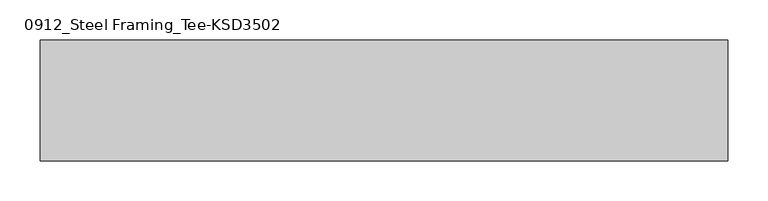
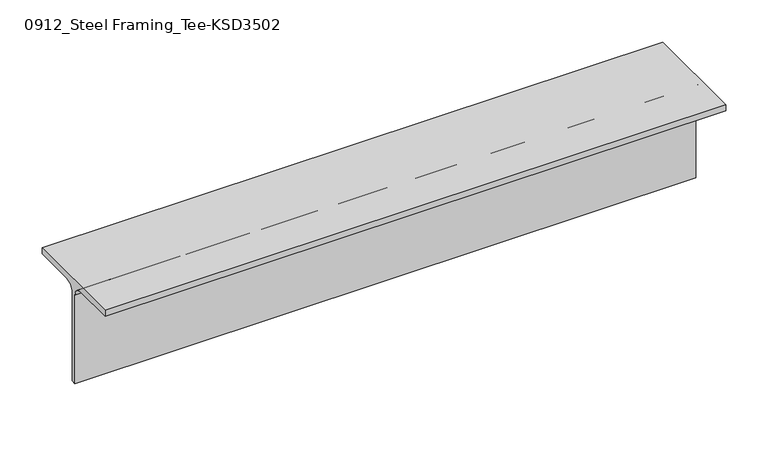
"""IFC4 building model written with IfcOpenShell, lengths in millimetres: member geometry, 0912_Steel Framing_Tee-KSD3502 : H_SB_ASB_CT-150x150x6.5x9."""

from ifc_helpers import new_model, si_unit, point, frame, frame_2d, origin, place, context, project, spatial, polyline, circle_curve, trimmed, segment, composite_curve, outline, extrude, source, transform, mapped, element, save


def member_0912_steel_framing_tee_ksd3502_a741d792(model_context):
    return source(origin(), model_context, "Body", "SweptSolid", [
        extrude(outline(composite_curve([segment(polyline([(75.0, 75.0), (75.0, 66.0), (16.25, 66.0)]), True, "CONTINUOUS"), segment(trimmed(circle_curve(frame_2d((16.25, 53.0)), 13.0), [point((16.25, 66.0))], [point((3.25, 53.0))], True, "CARTESIAN"), True, "CONTINUOUS"), segment(polyline([(3.25, 53.0), (3.25, -75.0), (-3.25, -75.0), (-3.25, 53.0)]), True, "CONTINUOUS"), segment(trimmed(circle_curve(frame_2d((-16.25, 53.0)), 13.0), [point((-3.25, 53.0))], [point((-16.25, 66.0))], True, "CARTESIAN"), True, "CONTINUOUS"), segment(polyline([(-16.25, 66.0), (-75.0, 66.0), (-75.0, 75.0), (75.0, 75.0)]), True, "CONTINUOUS")], self_intersect=False)), frame((-500.0, 0.0, 0.0), z_axis=(1.0, 0.0, 0.0), x_axis=(0.0, 1.0, 0.0)), (0.0, 0.0, 1.0), 853.0),
    ])


if __name__ == "__main__":
    model = new_model("IFC4")
    model_context = context("Model", 3, world=origin())
    ifc_project = project(units=[si_unit("LENGTHUNIT", "METRE", prefix="MILLI")], contexts=[model_context])
    site = spatial("IfcSite", under=ifc_project)
    building = spatial("IfcBuilding", under=site)
    placement = place(None, origin())
    member_0912_steel_framing_tee_ksd3502_shape = member_0912_steel_framing_tee_ksd3502_a741d792(model_context)
    element("IfcMember", 1, ObjectType="0912_Steel Framing_Tee-KSD3502 : H_SB_ASB_CT-150x150x6.5x9", at=placement, inside=building, context=model_context, shape_type="MappedRepresentation", body=[
        mapped(member_0912_steel_framing_tee_ksd3502_shape, transform((0.0, 0.0, 0.0), x_axis=(1.0, 0.0, 0.0), y_axis=(0.0, 1.0, 0.0), z_axis=(0.0, 0.0, 1.0))),
    ])
    save(model, "model.ifc")

# Revit data of these elements
# Type "0912_Steel Framing_Tee-KSD3502 : H_SB_ASB_CT-150x150x6.5x9"
#   H_WM Code_1 = "S01AA003-00001 | Main Steel Structure Fabrication Work | Shelter/Building | Light Steel - Standard (30KG/M>Weight) | Material: (   )"
#   H_WM Code_2 = "S03AA029-00001 | Main Steel Structure Erection Work | Shelter/Building | Light Steel (30KG/M>Weight) | Material: (   )"
#   H_WM Code_3 = "S01AA010-00001 | Main Steel Structure Fabrication Work | Shelter/Building | Steel Painting/Coating | for Non-Fireproofed Steel Surface, Surface Preparation, Primer, Second & Final Coat | Material: (   )"
#   H_Q'ty Cal Type Tag = "SB-Q2"
#   Width = 15.0 cm
#   Web Thickness = 0.65 cm
#   Web Fillet = 1.3 cm
#   Section Area = 23.39 cm²
#   Perimeter = 0.60 m²/m
#   Nominal Weight = 18.40 kgf/m
#   Height = 15.0 cm
#   Flange Thickness = 0.9 cm
#   Centroid Vertical = 7.5 cm
#   Centroid Horizontal = 7.5 cm
#   Length [instance default] = 1.5000 m
#   Structural Material [instance default] = Steel, 45-345
#   Warping Constant = (empty or 0)
#   Torsional Moment of Inertia = 0
#   Section Name Key = ""
#   Plastic Modulus weak axis = 0
#   Plastic Modulus strong axis = 0
#   Moment of Inertia weak axis = 0
#   Moment of Inertia strong axis = 0
#   Elastic Modulus weak axis = 0
#   Elastic Modulus strong axis = 0
#   Bolt Spacing = 0
#   Assembly Code = ""
# Element 1 (IfcMember, "0912_Steel Framing_Tee-KSD3502 : H_SB_ASB_CT-150x150x6.5x9")
#   Structural Material = none
# Materials
#   "Steel, 45-345": class "Metal", colour RGB 189 187 185, transparency 0, Description = "Steel 345 MPa", Cost = 0
